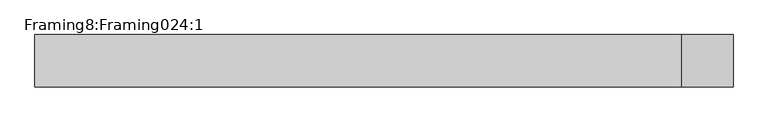
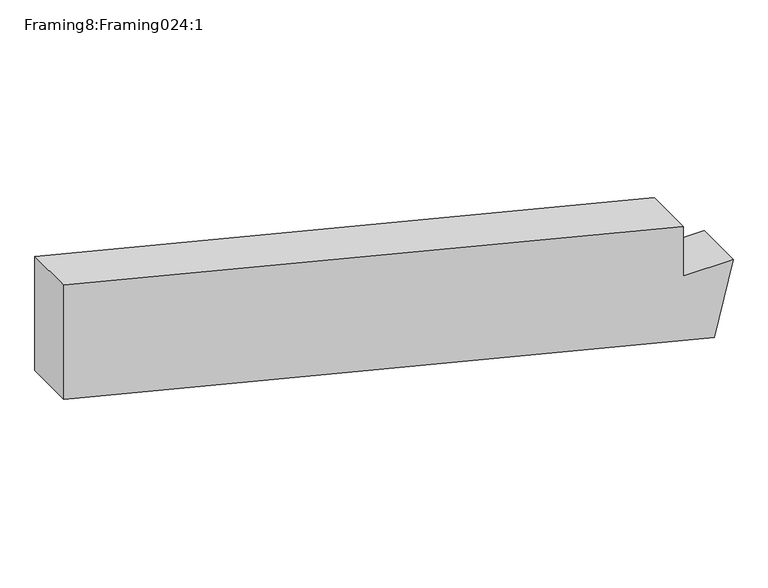
"""IFC4 building model written with IfcOpenShell, lengths in millimetres: proxy geometry, Framing8:Framing024:1 : Framing8:Framing024:286352."""

from ifc_helpers import new_model, si_unit, frame, origin, place, context, project, spatial, polyline, outline, extrude, source, transform, mapped, element, save


def framing8_framing024_1_e8013b78(model_context):
    return source(origin(), model_context, "Body", "SweptSolid", [
        extrude(outline(polyline([(111678.1362587, 15130.8894286), (111908.8006385, 15187.4083443), (111908.8006385, 15036.8413595), (112067.5842581, 15036.8413595), (112537.4873042, 13157.0903708), (112170.6516785, 13157.0903708), (111678.1362587, 15130.8894286)])), frame((0.0, -13445.349577, 0.0), z_axis=(0.0, 1.0, 0.0), x_axis=(0.0, 0.0, 1.0)), (0.0, 0.0, 1.0), 152.4),
    ])


if __name__ == "__main__":
    model = new_model("IFC4")
    model_context = context("Model", 3, world=origin())
    ifc_project = project(units=[si_unit("LENGTHUNIT", "METRE", prefix="MILLI")], contexts=[model_context])
    site = spatial("IfcSite", under=ifc_project)
    building = spatial("IfcBuilding", under=site)
    placement = place(None, origin())
    framing8_framing024_1_shape = framing8_framing024_1_e8013b78(model_context)
    element("IfcBuildingElementProxy", 1, Name="Framing8:Framing024:1 : Framing8:Framing024:286352", ObjectType="Framing8:Framing024:1 : Framing8:Framing024:286352", at=placement, inside=building, context=model_context, shape_type="MappedRepresentation", body=[
        mapped(framing8_framing024_1_shape, transform((0.0, 0.0, 0.0), x_axis=(1.0, 0.0, 0.0), y_axis=(0.0, 1.0, 0.0), z_axis=(0.0, 0.0, 1.0))),
    ])
    save(model, "model.ifc")

# Revit data of these elements
# Type "Framing8:Framing024:1 : Framing8:Framing024:286352"
#   NameOverride = "Framing8:Framing024:286352"
#   ObjectTypeOverride = "Framing8:Framing024"
#   Reference = "Framing024"
#   Category = "Generic Models"
#   Tag = "286352"
# Element 1 (IfcBuildingElementProxy, "Framing8:Framing024:1 : Framing8:Framing024:286352")
#   Materials on its faces: "WOOD FRAMING (SEE STRUCT DWGS)"
# Materials
#   "WOOD FRAMING (SEE STRUCT DWGS)": class "Unassigned", colour RGB 224 188 168, transparency 0, Cost = 0
